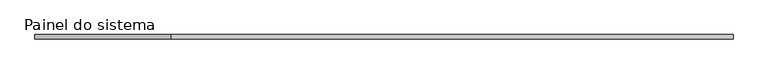
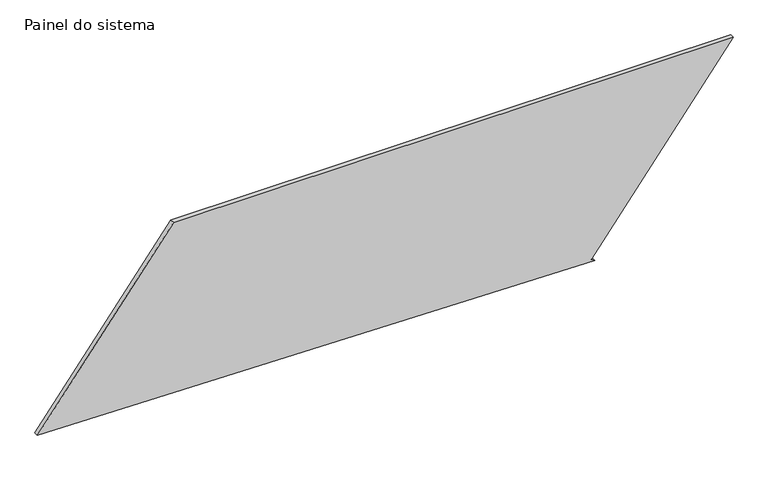
"""IFC4 building model written with IfcOpenShell, lengths in millimetres: plate geometry, Painel do sistema : Envidraçado."""

from ifc_helpers import new_model, si_unit, frame, origin, place, context, project, spatial, polyline, outline, extrude, source, transform, mapped, element, save


def painel_do_sistema_f4725ed1(model_context):
    return source(origin(), model_context, "Body", "SweptSolid", [
        extrude(outline(polyline([(0.0, 1200.8191461), (15.2063352, 1180.9755736), (1077.6041019, 1995.1019854), (1077.6041019, -1214.5379975), (59.0037648, -1995.1019854), (0.0, 1200.8191461)])), frame((0.0, 24.5, 0.0), z_axis=(0.0, 1.0, 0.0), x_axis=(0.0, 0.0, 1.0)), (0.0, 0.0, 1.0), 25.0),
    ])


if __name__ == "__main__":
    model = new_model("IFC4")
    model_context = context("Model", 3, world=origin())
    ifc_project = project(units=[si_unit("LENGTHUNIT", "METRE", prefix="MILLI")], contexts=[model_context])
    site = spatial("IfcSite", under=ifc_project)
    building = spatial("IfcBuilding", under=site)
    placement = place(None, origin())
    painel_do_sistema_shape = painel_do_sistema_f4725ed1(model_context)
    element("IfcPlate", 1, ObjectType="Painel do sistema : Envidraçado", at=placement, inside=building, context=model_context, shape_type="MappedRepresentation", body=[
        mapped(painel_do_sistema_shape, transform((0.0, 0.0, 0.0), x_axis=(1.0, 0.0, 0.0), y_axis=(0.0, 1.0, 0.0), z_axis=(0.0, 0.0, 1.0))),
    ])
    save(model, "model.ifc")

# Revit data of these elements
# Type "Painel do sistema : Envidraçado"
#   Construction Type Id = "GSP4R"
#   Analytic Construction = "Vidraça única Pilkington 1/8 pol"
#   Visual Light Transmittance = 0.9
#   Solar Heat Gain Coefficient = 0.86
#   Heat Transfer Coefficient (U) = 6.7069 W/(m²·K)
# Element 1 (IfcPlate, "Painel do sistema : Envidraçado")
#   Materials on its faces: "Vidro"
# Materials
#   "Vidro": class "Vidro", colour RGB 0 128 192, transparency 0.9, Description = "Vidro de sílica", Cost = 0
